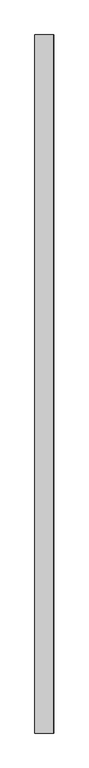
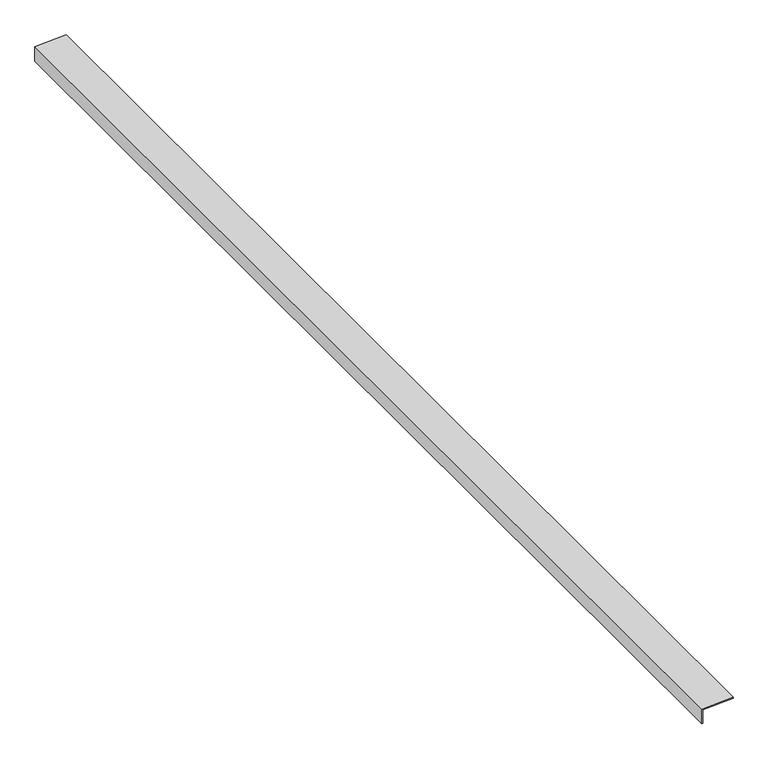
"""IFC4 building model written with IfcOpenShell, lengths in millimetres: proxy geometry, Generic Models 7:Generic Models 1:8:Generic Models 1:8 : Generic Models 7:Generic Models 1:337419:51 : Generic Models 7:Generic Models 1:8:Generic Models 1:8 : Generic Models 7:Generic Models 1:337419:315935."""

from ifc_helpers import new_model, si_unit, frame, origin, place, context, project, spatial, polyline, outline, extrude, source, transform, mapped, element, save


def generic_models_68df8388(model_context):
    return source(origin(), model_context, "Body", "SweptSolid", [
        extrude(outline(polyline([(3665.1571615, 560245.7438789), (3712.5900973, 560245.7438789), (3716.7350684, 560345.2231854), (3720.2423053, 560345.0770505), (3715.9571615, 560242.2335989), (3665.1571615, 560242.2335989), (3665.1571615, 560245.7438789)])), frame((0.0, -546983.9913841, 0.0), z_axis=(0.0, 1.0, 0.0), x_axis=(0.0, 0.0, 1.0)), (0.0, 0.0, 1.0), 3800.475),
    ])


if __name__ == "__main__":
    model = new_model("IFC4")
    model_context = context("Model", 3, world=origin())
    ifc_project = project(units=[si_unit("LENGTHUNIT", "METRE", prefix="MILLI")], contexts=[model_context])
    site = spatial("IfcSite", under=ifc_project)
    building = spatial("IfcBuilding", under=site)
    placement = place(None, origin())
    generic_models_shape = generic_models_68df8388(model_context)
    element("IfcBuildingElementProxy", 1, Name="Generic Models 7:Generic Models 1:8:Generic Models 1:8 : Generic Models 7:Generic Models 1:337419:51 : Generic Models 7:Generic Models 1:8:Generic Models 1:8 : Generic Models 7:Generic Models 1:337419:315935", ObjectType="Generic Models 7:Generic Models 1:8:Generic Models 1:8 : Generic Models 7:Generic Models 1:337419:51 : Generic Models 7:Generic Models 1:8:Generic Models 1:8 : Generic Models 7:Generic Models 1:337419:315935", at=placement, inside=building, context=model_context, shape_type="MappedRepresentation", body=[
        mapped(generic_models_shape, transform((0.0, 0.0, 0.0), x_axis=(1.0, 0.0, 0.0), y_axis=(0.0, 1.0, 0.0), z_axis=(0.0, 0.0, 1.0))),
    ])
    save(model, "model.ifc")

# Revit data of these elements
# Type "Generic Models 7:Generic Models 1:8:Generic Models 1:8 : Generic Models 7:Generic Models 1:337419:51 : Generic Models 7:Generic Models 1:8:Generic Models 1:8 : Generic Models 7:Generic Models 1:337419:315935"
#   NameOverride = "Generic Models 7:Generic Models 1:8:Generic Models 1:8 : Generic Models 7:Generic Models 1:337419:315935"
#   ObjectTypeOverride = "Generic Models 1:8 : Generic Models 7:Generic Models 1:337419"
#   Reference = "Generic Models 1"
#   Tag = "315935"
# Element 1 (IfcBuildingElementProxy, "Generic Models 7:Generic Models 1:8:Generic Models 1:8 : Generic Models 7:Generic Models 1:337419:51 : Generic Models 7:Generic Models 1:8:Generic Models 1:8 : Generic Models 7:Generic Models 1:337419:315935")
#   Materials on its faces: "11 GA. ALUM. BRAKE METAL (ALIGN WITH B.M. @ STOREFRONT/RESIN/POLYCARBONATE)"
# Materials
#   "11 GA. ALUM. BRAKE METAL (ALIGN WITH B.M. @ STOREFRONT/RESIN/POLYCARBONATE)": class "Unassigned", colour RGB 210 209 208, transparency 0, Cost = 0
